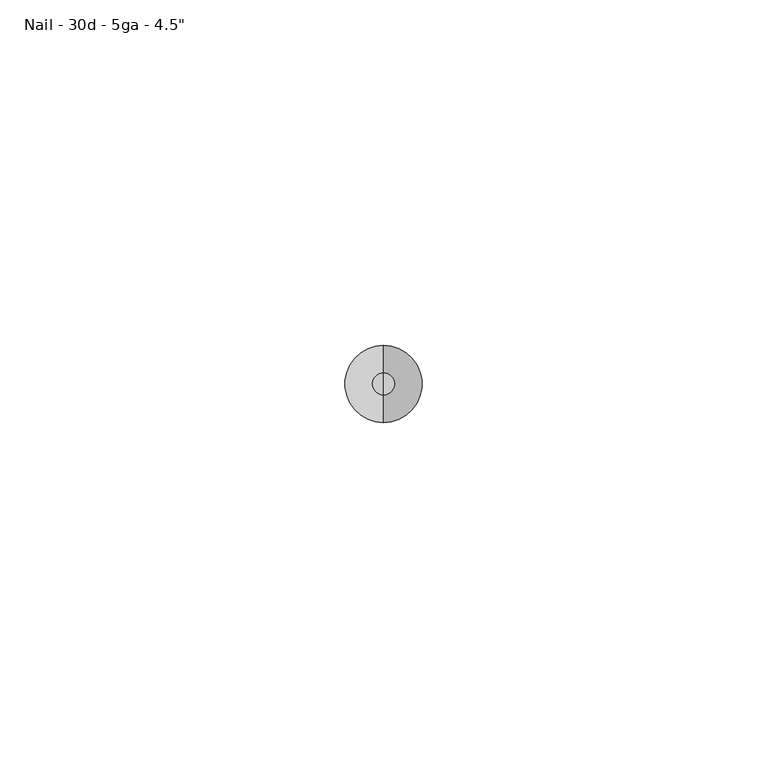
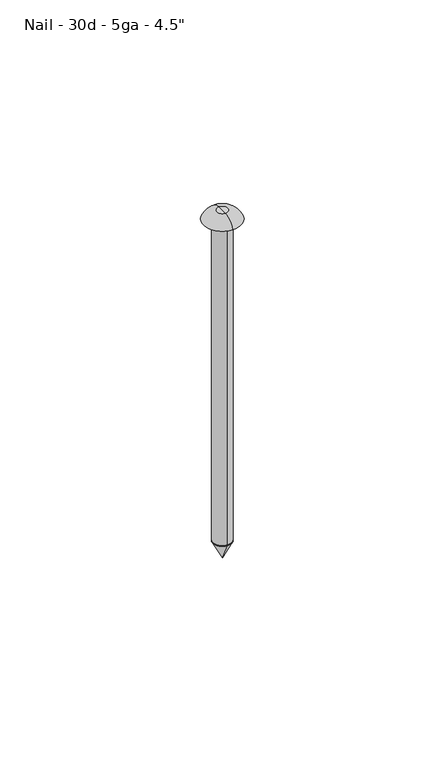
"""IFC4 building model written with IfcOpenShell, lengths in millimetres: fastener geometry."""

from ifc_helpers import new_model, si_unit, point, frame, origin, origin_2d, place, context, project, spatial, polyline, circle_curve, ellipse_curve, trimmed, segment, composite_curve, outline, extrude, source, transform, mapped, element, save
from ifc_brep_helpers import plane_surface, revolved_surface, advanced_brep


def fastener_30999ae7(model_context):
    return source(origin(), model_context, "Body", "SolidModel", [
        advanced_brep(
        [(0.0, -2.794, -101.6), (0.0, 2.794, -101.6), (0.0, 0.0, -101.6), (0.0, 0.0, -107.188)],
        [
            (0, 1, circle_curve(frame((0.0, 0.0, -101.6), z_axis=(0.0, 0.0, 1.0), x_axis=(0.0, 1.0, 0.0)), 2.794)),
            (1, 2),
            (2, 0),
            (1, 0, circle_curve(frame((0.0, 0.0, -101.6), z_axis=(0.0, 0.0, 1.0), x_axis=(0.0, 1.0, 0.0)), 2.794)),
            (3, 1),
            (0, 3),
        ],
        [
            plane_surface(frame((0.0, 0.0, -101.6), z_axis=(0.0, 0.0, 1.0), x_axis=(0.0, 1.0, 0.0))),
            revolved_surface(polyline([(0.0, 2.794, -101.6), (0.0, 0.0, -107.188)]), (0.0, 0.0, -103.0840259), (0.0, 0.0, -1.0)),
        ],
        [
            (0, [[1, 2, 3]]),
            (0, [[4, -3, -2]]),
            (1, [[5, -1, 6]]),
            (1, [[-6, -4, -5]]),
        ],
    ),
        advanced_brep(
        [(0.0, 5.588, 0.0), (0.0, -5.588, 0.0), (0.0, 0.0, 0.0), (0.0, 0.0, 2.794), (0.0, -1.5875, 2.794), (0.0, 1.5875, 2.794)],
        [
            (0, 1, circle_curve(frame((0.0, 0.0, 0.0), z_axis=(0.0, 0.0, -1.0), x_axis=(0.0, -1.0, 0.0)), 5.588)),
            (1, 2),
            (2, 0),
            (1, 0, circle_curve(frame((0.0, 0.0, 0.0), z_axis=(0.0, 0.0, -1.0), x_axis=(0.0, -1.0, 0.0)), 5.588)),
            (3, 4),
            (4, 5, circle_curve(frame((0.0, 0.0, 2.794), z_axis=(0.0, 0.0, 1.0), x_axis=(0.0, -1.0, 0.0)), 1.5875)),
            (5, 3),
            (5, 4, circle_curve(frame((0.0, 0.0, 2.794), z_axis=(0.0, 0.0, 1.0), x_axis=(0.0, -1.0, 0.0)), 1.5875)),
            (4, 1, circle_curve(frame((0.0, -1.5875, -1.4669943), z_axis=(1.0, 0.0, 0.0), x_axis=(0.0, -1.0, 0.0)), 4.2609943)),
            (0, 5, circle_curve(frame((0.0, 1.5875, -1.4669943), z_axis=(1.0, 0.0, 0.0), x_axis=(0.0, 1.0, 0.0)), 4.2609943)),
        ],
        [
            plane_surface(frame((0.0, 0.0, 0.0), z_axis=(0.0, 0.0, -1.0), x_axis=(0.0, -1.0, 0.0))),
            plane_surface(frame((0.0, 0.0, 2.794), z_axis=(0.0, 0.0, 1.0), x_axis=(0.0, -1.0, 0.0))),
            revolved_surface(trimmed(ellipse_curve(frame((0.0, -1.5875, -1.4669943), z_axis=(-1.0, 0.0, 0.0), x_axis=(0.0, -1.0, 0.0)), 4.2609943, 4.2609943), [point((0.0, -5.588, 0.0))], [point((0.0, -1.5875, 2.794))], True, "CARTESIAN"), (0.0, 0.0, 1.4840259), (0.0, 0.0, 1.0)),
        ],
        [
            (0, [[1, 2, 3]]),
            (0, [[4, -3, -2]]),
            (1, [[5, 6, 7]]),
            (1, [[-7, 8, -5]]),
            (2, [[-6, 9, -1, 10]]),
            (2, [[-8, -10, -4, -9]]),
        ],
    ),
        extrude(outline(composite_curve([segment(trimmed(circle_curve(origin_2d(), 2.794), [point((0.0, -2.794))], [point((0.0, 2.794))], False, "CARTESIAN"), True, "CONTINUOUS"), segment(trimmed(circle_curve(origin_2d(), 2.794), [point((0.0, 2.794))], [point((0.0, -2.794))], False, "CARTESIAN"), True, "CONTINUOUS")], self_intersect=False)), frame((0.0, 0.0, -101.6), z_axis=(0.0, 0.0, 1.0), x_axis=(1.0, 0.0, 0.0)), (0.0, 0.0, 1.0), 101.6),
    ])


if __name__ == "__main__":
    model = new_model("IFC4")
    model_context = context("Model", 3, world=origin())
    ifc_project = project(units=[si_unit("LENGTHUNIT", "METRE", prefix="MILLI")], contexts=[model_context])
    site = spatial("IfcSite", under=ifc_project)
    building = spatial("IfcBuilding", under=site)
    placement = place(None, origin())
    fastener_shape = fastener_30999ae7(model_context)
    element("IfcFastener", 1, ObjectType="060523 - W_P_C - Fastenings - Generic : Nail - 30d - 5ga - 4.5\"", at=placement, inside=building, context=model_context, shape_type="MappedRepresentation", body=[
        mapped(fastener_shape, transform((0.0, 0.0, 0.0), x_axis=(1.0, 0.0, 0.0), y_axis=(0.0, 1.0, 0.0), z_axis=(0.0, 0.0, 1.0))),
    ])
    save(model, "model.ifc")

# Revit data of these elements
# Type "060523 - W_P_C - Fastenings - Generic : Nail - 30d - 5ga - 4.5\""
#   Washer_Thickness = 0' - 0.00333"
#   Washer Radius = 0' - 0.12"
#   Washer Offset - Head = 0' - 0"
#   Washer Offset = 0' - 0"
#   Thickness_of_Substrate [instance default] = 0' - 1"
#   Side = 0' - 0 37/64"
#   Radius = 0' - 0.11"
#   Length [instance default] = 0' - 4 1/2"
#   Head Size = 0' - 1"
#   Head Radius = 0' - 0 1/2"
#   Head Height = 0' - 0.01"
#   Double Diameter = 0' - 0.44"
#   Diameter = 0' - 0.22"
#   Default Elevation = 4' - 0"
#   Washer_Nut_Visibility = no
#   Washer_Head_Visibility = no
#   Round_Head_Visibility = yes
#   Point Visibility = yes
#   Nut_Visibility = no
#   Hex_Head_Visiblilty = no
#   Washer Material = none
#   Bolt Material (Size) = AT SILL - FASTENER AT 24" O.C.
# Element 1 (IfcFastener, "060523 - W_P_C - Fastenings - Generic : Nail - 30d - 5ga - 4.5\"")
#   Length = 0' - 4"
#   Materials on its faces: "AT SILL - FASTENER AT 24\" O.C."
# Materials
#   "AT SILL - FASTENER AT 24\" O.C.": class "Generic", colour RGB 120 120 120, transparency 0, Cost = 0
